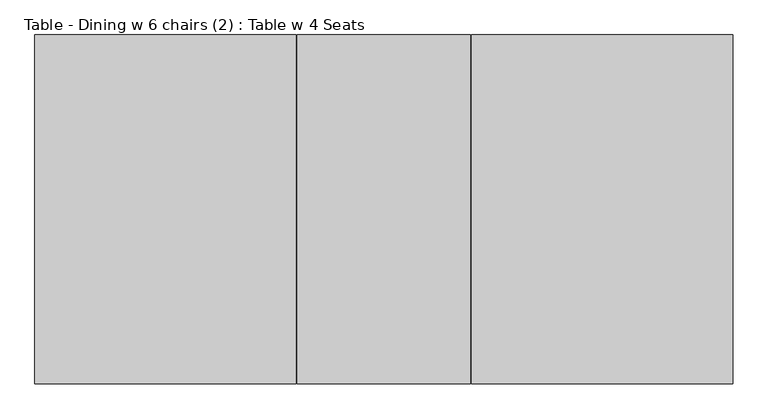
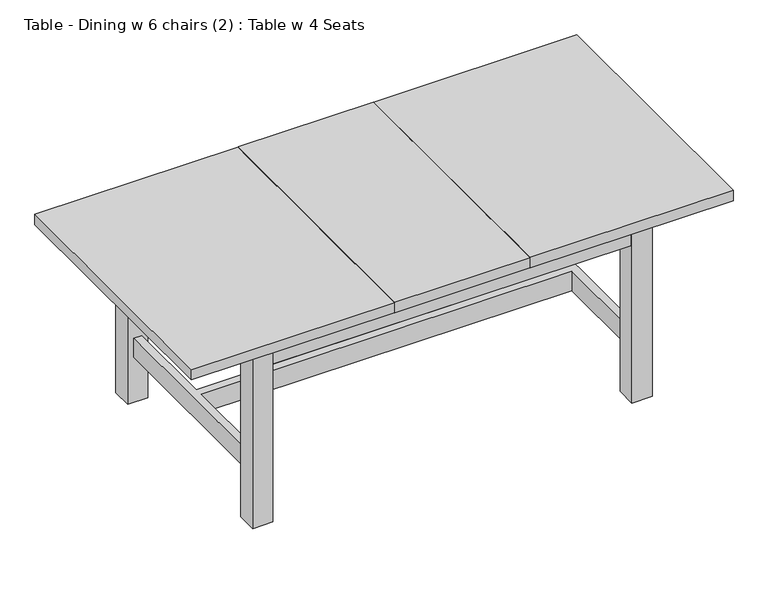
"""IFC4 building model written with IfcOpenShell, lengths in millimetres: furniture geometry, Table - Dining w 6 chairs (2) : Table w 4 Seats."""

from ifc_helpers import new_model, si_unit, frame, origin, origin_with_axes, place, context, project, spatial, polyline, outline, extrude, faceted_brep, source, transform, mapped, element, save


def table_dining_w_6_chairs_2_table_w_4_seats_080c21d9(model_context):
    return source(origin(), model_context, "Body", "SolidModel", [
        extrude(outline(polyline([(-544.3212781, 474.3546292), (780.6787219, 474.3546292), (780.6787219, 454.3546292), (-544.3212781, 454.3546292), (-544.3212781, 474.3546292)])), frame((0.0, 0.0, 610.0), z_axis=(0.0, 0.0, 1.0), x_axis=(1.0, 0.0, 0.0)), (0.0, 0.0, 1.0), 100.0),
        extrude(outline(polyline([(-611.8212781, -318.1453708), (-611.8212781, 406.8546292), (-591.8212781, 406.8546292), (-591.8212781, -318.1453708), (-611.8212781, -318.1453708)])), frame((0.0, 0.0, 610.0), z_axis=(0.0, 0.0, 1.0), x_axis=(1.0, 0.0, 0.0)), (0.0, 0.0, 1.0), 100.0),
        extrude(outline(polyline([(780.6787219, -385.6453708), (-544.3212781, -385.6453708), (-544.3212781, -365.6453708), (780.6787219, -365.6453708), (780.6787219, -385.6453708)])), frame((0.0, 0.0, 610.0), z_axis=(0.0, 0.0, 1.0), x_axis=(1.0, 0.0, 0.0)), (0.0, 0.0, 1.0), 100.0),
        extrude(outline(polyline([(848.1787219, 406.8546292), (848.1787219, -318.1453708), (828.1787219, -318.1453708), (828.1787219, 406.8546292), (848.1787219, 406.8546292)])), frame((0.0, 0.0, 610.0), z_axis=(0.0, 0.0, 1.0), x_axis=(1.0, 0.0, 0.0)), (0.0, 0.0, 1.0), 100.0),
        extrude(outline(polyline([(-566.8212781, -318.1453708), (-596.8212781, -318.1453708), (-596.8212781, 406.8546292), (-566.8212781, 406.8546292), (-566.8212781, 59.3546292), (803.1787219, 59.3546292), (803.1787219, 406.8546292), (833.1787219, 406.8546292), (833.1787219, -318.1453708), (803.1787219, -318.1453708), (803.1787219, 29.3546292), (-566.8212781, 29.3546292), (-566.8212781, -318.1453708)])), frame((0.0, 0.0, 175.0), z_axis=(0.0, 0.0, 1.0), x_axis=(1.0, 0.0, 0.0)), (0.0, 0.0, 1.0), 75.0),
        extrude(outline(polyline([(-544.3212781, -393.1453708), (-619.3212781, -393.1453708), (-619.3212781, -318.1453708), (-544.3212781, -318.1453708), (-544.3212781, -393.1453708)])), origin_with_axes(), (0.0, 0.0, 1.0), 710.0),
        extrude(outline(polyline([(780.6787219, 481.8546292), (855.6787219, 481.8546292), (855.6787219, 406.8546292), (780.6787219, 406.8546292), (780.6787219, 481.8546292)])), origin_with_axes(), (0.0, 0.0, 1.0), 710.0),
        extrude(outline(polyline([(780.6787219, -318.1453708), (855.6787219, -318.1453708), (855.6787219, -393.1453708), (780.6787219, -393.1453708), (780.6787219, -318.1453708)])), origin_with_axes(), (0.0, 0.0, 1.0), 710.0),
        extrude(outline(polyline([(-544.3212781, 481.8546292), (-544.3212781, 406.8546292), (-619.3212781, 406.8546292), (-619.3212781, 481.8546292), (-544.3212781, 481.8546292)])), origin_with_axes(), (0.0, 0.0, 1.0), 710.0),
        faceted_brep([(1118.1787219, -455.6453708, 750.0), (1118.1787219, 544.3546292, 750.0), (369.6787219, 544.3546292, 750.0), (369.6787219, -455.6453708, 750.0), (-881.8212781, 544.3546292, 750.0), (-881.8212781, -455.6453708, 750.0), (-133.3212781, -455.6453708, 750.0), (-133.3212781, 544.3546292, 750.0), (366.6787219, 544.3546292, 750.0), (-130.3212781, 544.3546292, 750.0), (-130.3212781, -455.6453708, 750.0), (366.6787219, -455.6453708, 750.0), (-881.8212781, -455.6453708, 710.0), (-881.8212781, 544.3546292, 710.0), (-133.3212781, 544.3546292, 710.0), (-131.8212781, 542.8546292, 710.0), (-130.3212781, 544.3546292, 710.0), (366.6787219, 544.3546292, 710.0), (368.1787219, 542.8546292, 710.0), (369.6787219, 544.3546292, 710.0), (1118.1787219, 544.3546292, 710.0), (1118.1787219, -455.6453708, 710.0), (369.6787219, -455.6453708, 710.0), (368.1787219, -454.1453708, 710.0), (366.6787219, -455.6453708, 710.0), (-130.3212781, -455.6453708, 710.0), (-131.8212781, -454.1453708, 710.0), (-133.3212781, -455.6453708, 710.0), (-131.8212781, 542.8546292, 748.5), (368.1787219, 542.8546292, 748.5), (-131.8212781, -454.1453708, 748.5), (368.1787219, -454.1453708, 748.5)], [[[0, 1, 2, 3]], [[4, 5, 6, 7]], [[8, 9, 10, 11]], [[12, 13, 14, 15, 16, 17, 18, 19, 20, 21, 22, 23, 24, 25, 26, 27]], [[1, 0, 21, 20]], [[9, 8, 17, 16]], [[1, 20, 19, 2]], [[13, 4, 7, 14]], [[5, 4, 13, 12]], [[11, 10, 25, 24]], [[21, 0, 3, 22]], [[5, 12, 27, 6]], [[15, 28, 9, 16]], [[28, 15, 14, 7]], [[18, 29, 2, 19]], [[29, 18, 17, 8]], [[9, 28, 30, 10]], [[28, 7, 6, 30]], [[2, 29, 31, 3]], [[29, 8, 11, 31]], [[10, 30, 26, 25]], [[30, 6, 27, 26]], [[3, 31, 23, 22]], [[31, 11, 24, 23]]]),
    ])


if __name__ == "__main__":
    model = new_model("IFC4")
    model_context = context("Model", 3, world=origin())
    ifc_project = project(units=[si_unit("LENGTHUNIT", "METRE", prefix="MILLI")], contexts=[model_context])
    site = spatial("IfcSite", under=ifc_project)
    building = spatial("IfcBuilding", under=site)
    placement = place(None, origin())
    table_dining_w_6_chairs_2_table_w_4_seats_shape = table_dining_w_6_chairs_2_table_w_4_seats_080c21d9(model_context)
    element("IfcFurniture", 1, ObjectType="Table - Dining w 6 chairs (2) : Table w 4 Seats", at=placement, inside=building, context=model_context, shape_type="MappedRepresentation", body=[
        mapped(table_dining_w_6_chairs_2_table_w_4_seats_shape, transform((0.0, 0.0, 0.0), x_axis=(1.0, 0.0, 0.0), y_axis=(0.0, 1.0, 0.0), z_axis=(0.0, 0.0, 1.0))),
    ])
    save(model, "model.ifc")

# Revit data of these elements
# Project information
#   Project Status = "Project Status"
#   Client Name = "Revit Project"
#   Project Address = "Enter address here"
#   Project Name = "Two Storey Residence"
#   Project Number = "P.01"
# Type "Table - Dining w 6 chairs (2) : Table w 4 Seats"
#   Keynote = "N"
#   Width = 1000 mm
#   Table Top Thickness = 40 mm
#   Table Height = 750 mm
#   Length = 2000 mm
#   Leg Width = 75 mm
#   Leg Spacing Width = 800 mm
#   Leg Spacing Length = 1400 mm
#   Chair Side Spacing = 700 mm
#   Centre Piece = 500 mm
#   Vis - End Chairs = no
#   Material Table = Wood - Birch
#   Material Chair Structure = Wood - Birch
#   Material Chair Covering = Fabric - Beige
# Element 1 (IfcFurniture, "Table - Dining w 6 chairs (2) : Table w 4 Seats")
#   Materials on its faces: "Wood - Birch"
# Materials
#   "Wood - Birch": class "Wood", colour RGB 224 178 126, transparency 0
#   "Fabric - Beige": class "Fabric", colour RGB 231 227 195, transparency 0
